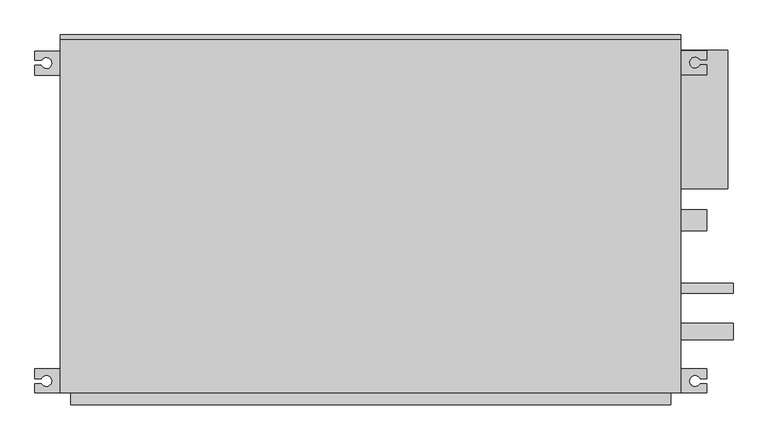
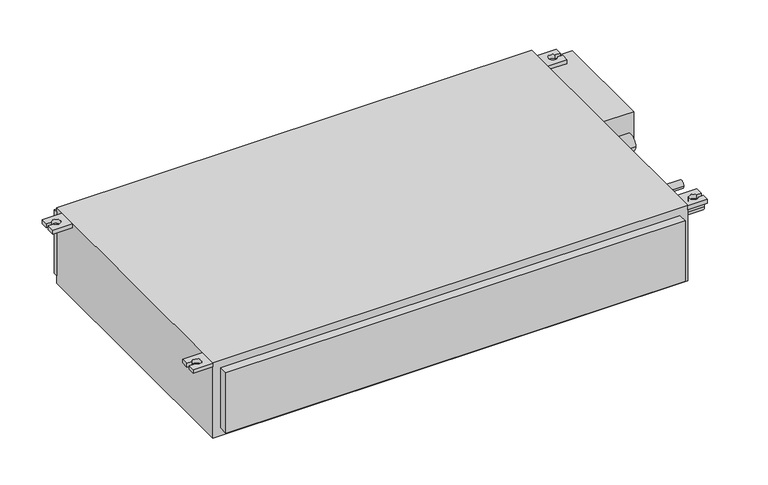
"""IFC4 building model written with IfcOpenShell, lengths in millimetres: proxy geometry, PEFY-P-NMSU-E_Low_Profile_Ducted : PEFY-P24NMSU-E."""

import ifcopenshell
import ifcopenshell.guid

model = None  # the IFC model being written
_history = None  # IfcOwnerHistory: only IFC2X3 demands one
_inside = {}  # id of a spatial element -> (the spatial element, [elements in it])
_under = {}  # id of a project, library or spatial element -> (it, [spatial elements below it])
_declared = {}  # id of a project -> (the project, [libraries it declares])
_typed = {}  # id of a type object -> (the type object, [elements of that type])
_made_of = {}  # id of a material, layer set ... -> (it, [elements and type objects made of it])


def new_model(schema):
    """Start an empty IFC model of exactly this schema.

    Asked for "IFC4X3", IfcOpenShell would pick the latest addendum, in which some entities
    have other attributes; the version numbers below select the first issue.
    IFC2X3 requires an IfcOwnerHistory on every rooted entity: one is made here for all.
    """
    global model, _history
    if schema == "IFC4X3":
        model = ifcopenshell.file(schema_version=(4, 3, 0, 0))
    else:
        model = ifcopenshell.file(schema=schema)
    _inside.clear()
    _under.clear()
    _declared.clear()
    _typed.clear()
    _made_of.clear()
    _history = None
    if model.schema == "IFC2X3":
        org = make("IfcOrganization", Name="unknown")
        user = make(
            "IfcPersonAndOrganization",
            ThePerson=make("IfcPerson", FamilyName="unknown"),
            TheOrganization=org,
        )
        app = make(
            "IfcApplication",
            ApplicationDeveloper=org,
            Version="unknown",
            ApplicationFullName="unknown",
            ApplicationIdentifier="unknown",
        )
        _history = make(
            "IfcOwnerHistory",
            OwningUser=user,
            OwningApplication=app,
            ChangeAction="ADDED",
            CreationDate=0,
        )
    return model


def make(cls, **values):
    """One entity of the class cls with the attributes given. An attribute that is None is left unset."""
    return model.create_entity(
        cls, **{name: value for name, value in values.items() if value is not None}
    )


def rooted(cls, **values):
    """An entity with a GlobalId (a new one), such as an element, a storey or a relation."""
    return make(cls, GlobalId=ifcopenshell.guid.new(), OwnerHistory=_history, **values)


def si_unit(unit_type, name, prefix=None):
    """IfcSIUnit, for example si_unit("LENGTHUNIT", "METRE", prefix="MILLI")."""
    return make("IfcSIUnit", UnitType=unit_type, Prefix=prefix, Name=name)


def assignment(units):
    """IfcUnitAssignment: the units of a project."""
    return None if units is None else make("IfcUnitAssignment", Units=units)


def point(xyz):
    """IfcCartesianPoint."""
    return None if xyz is None else make("IfcCartesianPoint", Coordinates=xyz)


def direction(xyz):
    """IfcDirection."""
    return None if xyz is None else make("IfcDirection", DirectionRatios=xyz)


def frame(location, z_axis=None, x_axis=None):
    """IfcAxis2Placement3D, a coordinate frame: its origin and axes. An axis left out is left unset."""
    return make(
        "IfcAxis2Placement3D",
        Location=point(location),
        Axis=direction(z_axis),
        RefDirection=direction(x_axis),
    )


def frame_2d(location, x_axis=None):
    """IfcAxis2Placement2D, a coordinate frame in the plane: its origin and x axis."""
    return make(
        "IfcAxis2Placement2D", Location=point(location), RefDirection=direction(x_axis)
    )


def origin():
    """The frame at (0, 0, 0) with its axes left unset."""
    return frame((0.0, 0.0, 0.0))


def origin_with_axes():
    """The frame at (0, 0, 0) with the z axis (0, 0, 1) and the x axis (1, 0, 0) written out."""
    return frame((0.0, 0.0, 0.0), z_axis=(0.0, 0.0, 1.0), x_axis=(1.0, 0.0, 0.0))


def place(relative_to, where):
    """IfcLocalPlacement: puts the frame where relative to a parent placement (None: the world)."""
    return make(
        "IfcLocalPlacement", PlacementRelTo=relative_to, RelativePlacement=where
    )


def context(
    kind, dimensions, precision=None, world=None, true_north=None, identifier=None
):
    """IfcGeometricRepresentationContext, for example the 3D "Model" context."""
    return make(
        "IfcGeometricRepresentationContext",
        ContextIdentifier=identifier,
        ContextType=kind,
        CoordinateSpaceDimension=dimensions,
        Precision=precision,
        WorldCoordinateSystem=world,
        TrueNorth=true_north,
    )


def project(units=None, contexts=None):
    """IfcProject with its units and contexts."""
    return rooted(
        "IfcProject",
        Name="project",
        RepresentationContexts=contexts,
        UnitsInContext=assignment(units),
    )


def spatial(cls, under=None, at=None, **own):
    """A site, building, storey or space (cls), placed at a placement, below another one or the project."""
    s = rooted(cls, ObjectPlacement=at, **own)
    if under is not None:
        _under.setdefault(under.id(), (under, []))[1].append(s)
    return s


def polyline(points):
    """IfcPolyline through the points."""
    return make("IfcPolyline", Points=[point(p) for p in points])


def circle_curve(where, radius):
    """IfcCircle in the frame where."""
    return make("IfcCircle", Position=where, Radius=radius)


def trimmed(basis, trim1, trim2, sense, master):
    """IfcTrimmedCurve: the piece of a basis curve between two trims."""
    return make(
        "IfcTrimmedCurve",
        BasisCurve=basis,
        Trim1=trim1,
        Trim2=trim2,
        SenseAgreement=sense,
        MasterRepresentation=master,
    )


def segment(curve, same_sense, transition):
    """IfcCompositeCurveSegment."""
    return make(
        "IfcCompositeCurveSegment",
        Transition=transition,
        SameSense=same_sense,
        ParentCurve=curve,
    )


def composite_curve(segments, self_intersect=None):
    """IfcCompositeCurve: segments joined end to end."""
    return make("IfcCompositeCurve", Segments=segments, SelfIntersect=self_intersect)


def outline(outer, holes=None, kind="AREA"):
    """IfcArbitraryClosedProfileDef: a profile drawn as a closed curve; with holes, ...WithVoids."""
    if holes is None:
        return make("IfcArbitraryClosedProfileDef", ProfileType=kind, OuterCurve=outer)
    return make(
        "IfcArbitraryProfileDefWithVoids",
        ProfileType=kind,
        OuterCurve=outer,
        InnerCurves=holes,
    )


def extrude(swept, where, along, depth):
    """IfcExtrudedAreaSolid: the profile swept, set in the frame where, extruded along a direction by depth."""
    return make(
        "IfcExtrudedAreaSolid",
        SweptArea=swept,
        Position=where,
        ExtrudedDirection=direction(along),
        Depth=depth,
    )


def shape(context_of_items, identifier, shape_type, items):
    """IfcShapeRepresentation: the items that make up one representation, for example the "Body"."""
    return make(
        "IfcShapeRepresentation",
        ContextOfItems=context_of_items,
        RepresentationIdentifier=identifier,
        RepresentationType=shape_type,
        Items=items,
    )


def source(mapping_origin, context_of_items, identifier, shape_type, items):
    """IfcRepresentationMap: a shape defined once, which mapped items show again and again."""
    return make(
        "IfcRepresentationMap",
        MappingOrigin=mapping_origin,
        MappedRepresentation=shape(context_of_items, identifier, shape_type, items),
    )


def transform(
    local_origin,
    x_axis=None,
    y_axis=None,
    z_axis=None,
    scale=None,
    scale2=None,
    scale3=None,
    uniform=True,
):
    """IfcCartesianTransformationOperator3D, or its non-uniform kind. x_axis, y_axis, z_axis: its Axis1, 2, 3."""
    if uniform:
        return make(
            "IfcCartesianTransformationOperator3D",
            Axis1=direction(x_axis),
            Axis2=direction(y_axis),
            LocalOrigin=point(local_origin),
            Scale=scale,
            Axis3=direction(z_axis),
        )
    return make(
        "IfcCartesianTransformationOperator3DnonUniform",
        Axis1=direction(x_axis),
        Axis2=direction(y_axis),
        LocalOrigin=point(local_origin),
        Scale=scale,
        Axis3=direction(z_axis),
        Scale2=scale2,
        Scale3=scale3,
    )


def mapped(mapping_source, mapping_target):
    """IfcMappedItem: shows the shape of a source again, moved by a transform."""
    return make(
        "IfcMappedItem", MappingSource=mapping_source, MappingTarget=mapping_target
    )


def made_of(thing, what):
    """Note that an element or type object is made of a material, layer set ...; save() writes the relation."""
    if what is not None:
        _made_of.setdefault(what.id(), (what, []))[1].append(thing)
    return thing


def element(
    cls,
    number,
    at=None,
    inside=None,
    cuts=None,
    type_object=None,
    material=None,
    context=None,
    identifier="Body",
    shape_type=None,
    held_by="IfcProductDefinitionShape",
    body=None,
    shapes=None,
    **own,
):
    """One element of the class cls, such as IfcWall. Its Tag is "e" and its number.

    at: its placement. inside: the storey or other place that contains it. cuts: it is an
    opening in that element (IfcRelVoidsElement). A single representation is given by context,
    identifier, shape_type and body (its items); several are given by shapes. held_by: the class
    of the entity that holds the representations. save() writes the other relations.
    """
    e = rooted(cls, Tag="e%d" % number, ObjectPlacement=at, **own)
    if body is not None:
        shapes = [shape(context, identifier, shape_type, body)]
    if shapes is not None:
        e.Representation = make(held_by, Representations=shapes)
    if inside is not None:
        _inside.setdefault(inside.id(), (inside, []))[1].append(e)
    if cuts is not None:
        rooted(
            "IfcRelVoidsElement", RelatingBuildingElement=cuts, RelatedOpeningElement=e
        )
    if type_object is not None:
        _typed.setdefault(type_object.id(), (type_object, []))[1].append(e)
    return made_of(e, material)


def aggregate(whole, parts):
    """IfcRelAggregates: a whole, such as a stair, and the parts it consists of."""
    return rooted("IfcRelAggregates", RelatingObject=whole, RelatedObjects=parts)


def save(model, path):
    """Write the relations noted so far, then the file.

    IfcRelAggregates (storeys below a building ...), IfcRelContainedInSpatialStructure (elements
    in a storey), IfcRelDefinesByType, IfcRelAssociatesMaterial and IfcRelDeclares: one each for
    every whole, place, type object, material and project.
    """
    for whole, parts in _under.values():
        aggregate(whole, parts)
    for where, things in _inside.values():
        rooted(
            "IfcRelContainedInSpatialStructure",
            RelatedElements=things,
            RelatingStructure=where,
        )
    for kind, things in _typed.values():
        rooted("IfcRelDefinesByType", RelatedObjects=things, RelatingType=kind)
    for what, things in _made_of.values():
        rooted("IfcRelAssociatesMaterial", RelatedObjects=things, RelatingMaterial=what)
    for by, libraries in _declared.values():
        rooted("IfcRelDeclares", RelatingContext=by, RelatedDefinitions=libraries)
    model.write(path)


def mechanical_equipment_2ac3c092(model_context):
    return source(origin(), model_context, "Body", "SweptSolid", [
        extrude(outline(composite_curve([segment(polyline([(-644.3, 282.0), (-644.3, 300.9759165), (-632.1454311, 300.9759165)]), True, "CONTINUOUS"), segment(trimmed(circle_curve(frame_2d((-622.2863556, 305.4254582)), 10.8166442), [point((-632.1454311, 300.9759165))], [point((-631.8387803, 310.5))], True, "CARTESIAN"), True, "CONTINUOUS"), segment(polyline([(-631.8387803, 310.5), (-644.3, 310.5), (-644.3, 328.0), (-595.3, 328.0), (-595.3, 282.0), (-644.3, 282.0)]), True, "CONTINUOUS")], self_intersect=False)), frame((0.0, 0.0, 188.55), z_axis=(0.0, 0.0, 1.0), x_axis=(1.0, 0.0, 0.0)), (0.0, 0.0, 1.0), 10.0),
        extrude(outline(composite_curve([segment(polyline([(-644.3, -281.0), (-595.3, -281.0), (-595.3, -327.0), (-644.3, -327.0), (-644.3, -309.5), (-631.8387803, -309.5)]), True, "CONTINUOUS"), segment(trimmed(circle_curve(frame_2d((-622.2863556, -304.4254582)), 10.8166442), [point((-631.8387803, -309.5))], [point((-632.1454311, -299.9759165))], True, "CARTESIAN"), True, "CONTINUOUS"), segment(polyline([(-632.1454311, -299.9759165), (-644.3, -299.9759165), (-644.3, -281.0)]), True, "CONTINUOUS")], self_intersect=False)), frame((0.0, 0.0, 188.55), z_axis=(0.0, 0.0, 1.0), x_axis=(1.0, 0.0, 0.0)), (0.0, 0.0, 1.0), 10.0),
        extrude(outline(composite_curve([segment(polyline([(644.3, 282.9429009), (595.3, 282.9429009), (595.3, 328.9429009), (644.3, 328.9429009), (644.3, 311.4429009), (631.8387803, 311.4429009)]), True, "CONTINUOUS"), segment(trimmed(circle_curve(frame_2d((622.2863556, 306.3683591)), 10.8166442), [point((631.8387803, 311.4429009))], [point((632.1454311, 301.9188174))], True, "CARTESIAN"), True, "CONTINUOUS"), segment(polyline([(632.1454311, 301.9188174), (644.3, 301.9188174), (644.3, 282.9429009)]), True, "CONTINUOUS")], self_intersect=False)), frame((0.0, 0.0, 188.55), z_axis=(0.0, 0.0, 1.0), x_axis=(1.0, 0.0, 0.0)), (0.0, 0.0, 1.0), 10.0),
        extrude(outline(composite_curve([segment(polyline([(644.3, -281.0), (644.3, -299.9759165), (632.1454311, -299.9759165)]), True, "CONTINUOUS"), segment(trimmed(circle_curve(frame_2d((622.2863556, -304.4254582)), 10.8166442), [point((632.1454311, -299.9759165))], [point((631.8387803, -309.5))], True, "CARTESIAN"), True, "CONTINUOUS"), segment(polyline([(631.8387803, -309.5), (644.3, -309.5), (644.3, -327.0), (595.3, -327.0), (595.3, -281.0), (644.3, -281.0)]), True, "CONTINUOUS")], self_intersect=False)), frame((0.0, 0.0, 188.55), z_axis=(0.0, 0.0, 1.0), x_axis=(1.0, 0.0, 0.0)), (0.0, 0.0, 1.0), 10.0),
        extrude(outline(polyline([(595.3, 350.04375), (-595.3, 350.04375), (-595.3, 359.5477547), (595.3, 359.5477547), (595.3, 350.04375)])), frame((0.0, 0.0, 20.0), z_axis=(0.0, 0.0, 1.0), x_axis=(1.0, 0.0, 0.0)), (0.0, 0.0, 1.0), 168.55),
        extrude(outline(composite_curve([segment(trimmed(circle_curve(frame_2d((4.0570991, 59.8)), 20.0), [point((-15.9429009, 59.8))], [point((24.0570991, 59.8))], False, "CARTESIAN"), True, "CONTINUOUS"), segment(trimmed(circle_curve(frame_2d((4.0570991, 59.8)), 20.0), [point((24.0570991, 59.8))], [point((-15.9429009, 59.8))], False, "CARTESIAN"), True, "CONTINUOUS")], self_intersect=False)), frame((595.3, 0.0, 0.0), z_axis=(1.0, 0.0, 0.0), x_axis=(0.0, 1.0, 0.0)), (0.0, 0.0, 1.0), 26.9863556),
        extrude(outline(composite_curve([segment(trimmed(circle_curve(frame_2d((4.0570991, 149.6)), 20.0), [point((-15.9429009, 149.6))], [point((24.0570991, 149.6))], False, "CARTESIAN"), True, "CONTINUOUS"), segment(trimmed(circle_curve(frame_2d((4.0570991, 149.6)), 20.0), [point((24.0570991, 149.6))], [point((-15.9429009, 149.6))], False, "CARTESIAN"), True, "CONTINUOUS")], self_intersect=False)), frame((595.3, 0.0, 0.0), z_axis=(1.0, 0.0, 0.0), x_axis=(0.0, 1.0, 0.0)), (0.0, 0.0, 1.0), 49.0),
        extrude(outline(composite_curve([segment(trimmed(circle_curve(frame_2d((-126.5596979, 100.0)), 9.5), [point((-136.0596979, 100.0))], [point((-117.0596979, 100.0))], False, "CARTESIAN"), True, "CONTINUOUS"), segment(trimmed(circle_curve(frame_2d((-126.5596979, 100.0)), 9.5), [point((-117.0596979, 100.0))], [point((-136.0596979, 100.0))], False, "CARTESIAN"), True, "CONTINUOUS")], self_intersect=False)), frame((595.3, 0.0, 0.0), z_axis=(1.0, 0.0, 0.0), x_axis=(0.0, 1.0, 0.0)), (0.0, 0.0, 1.0), 100.0),
        extrude(outline(composite_curve([segment(trimmed(circle_curve(frame_2d((-209.7540575, 100.0)), 15.9), [point((-225.6540575, 100.0))], [point((-193.8540575, 100.0))], False, "CARTESIAN"), True, "CONTINUOUS"), segment(trimmed(circle_curve(frame_2d((-209.7540575, 100.0)), 15.9), [point((-193.8540575, 100.0))], [point((-225.6540575, 100.0))], False, "CARTESIAN"), True, "CONTINUOUS")], self_intersect=False)), frame((595.3, 0.0, 0.0), z_axis=(1.0, 0.0, 0.0), x_axis=(0.0, 1.0, 0.0)), (0.0, 0.0, 1.0), 100.0),
        extrude(outline(polyline([(685.3, 330.0), (685.3, 64.0570991), (595.3, 64.0570991), (595.3, 330.0), (685.3, 330.0)])), frame((0.0, 0.0, 20.0), z_axis=(0.0, 0.0, 1.0), x_axis=(1.0, 0.0, 0.0)), (0.0, 0.0, 1.0), 159.8),
        extrude(outline(polyline([(575.3, -350.04375), (-575.3, -350.04375), (-575.3, -327.0), (575.3, -327.0), (575.3, -350.04375)])), frame((0.0, 0.0, 20.0), z_axis=(0.0, 0.0, 1.0), x_axis=(1.0, 0.0, 0.0)), (0.0, 0.0, 1.0), 159.8),
        extrude(outline(polyline([(-595.3, -327.0), (-595.3, 350.04375), (595.3, 350.04375), (595.3, -327.0), (-595.3, -327.0)])), origin_with_axes(), (0.0, 0.0, 1.0), 200.0),
    ])


if __name__ == "__main__":
    model = new_model("IFC4")
    model_context = context("Model", 3, world=origin())
    ifc_project = project(units=[si_unit("LENGTHUNIT", "METRE", prefix="MILLI")], contexts=[model_context])
    site = spatial("IfcSite", under=ifc_project)
    building = spatial("IfcBuilding", under=site)
    placement = place(None, origin())
    mechanical_equipment_shape = mechanical_equipment_2ac3c092(model_context)
    element("IfcBuildingElementProxy", 1, Name="PEFY-P-NMSU-E_Low_Profile_Ducted : PEFY-P24NMSU-E", ObjectType="PEFY-P-NMSU-E_Low_Profile_Ducted : PEFY-P24NMSU-E", at=placement, inside=building, context=model_context, shape_type="MappedRepresentation", body=[
        mapped(mechanical_equipment_shape, transform((0.0, 0.0, 0.0), x_axis=(1.0, 0.0, 0.0), y_axis=(0.0, 1.0, 0.0), z_axis=(0.0, 0.0, 1.0))),
    ])
    save(model, "model.ifc")

# Revit data of these elements
# Project information
#   Project Issue Date = "Issue Date"
#   Project Status = "Project Status"
#   Client Name = "Owner"
#   Project Address = "Enter address here"
#   Project Name = "Project Name"
#   Project Number = "Project Number"
# Type "PEFY-P-NMSU-E_Low_Profile_Ducted : PEFY-P24NMSU-E"
#   Subcategory = "HVAC"
#   Standard Air Filter = "Polypropylene Honeycomb"
#   Specification URL = "http://www.mrslim.com/customerCare/resources.asp"
#   Sound Pressure Levels (dB(A)) = "30-35-40"
#   SmartBIM Object Created By = "Reed Construction Data"
#   Refirigerant Pipe diameter (Liquid) = "3/8\""
#   Refirigerant Pipe diameter (Gas) = "5/8\""
#   Power Source = "208/230, 1, 60"
#   Power Consumption Heating = "0.10 kW"
#   Power Consumption Cooling = "0.12 kW"
#   Unit Weight (LBS) = "62"
#   Model = "PEFY-P24NMSU-E"
#   Manufacturer URL = "http://www.mrslim.com/customerCare/resources.asp"
#   Manufacturer = "Mitsubishi Electric"
#   Installation URL = "http://www.mrslim.com/customerCare/resources.asp"
#   Fan Motor Type = "DC Motor"
#   Fan Motor Output = "0.096 kW"
#   MCA = "1.57/1.73"
#   MOCP = "15 A"
#   E.S.P (In. W.G.) = ".02-.20"
#   Drainpipe Dimension = "1-1/4"
#   Description = "Ceiling Concealed Ducted Low Profile"
#   Condensate Lift Mechanism = "21-11/16\""
#   Coil Type = "Cross Fin"
#   Heating Capacity (BTU) = "27000"
#   Fan Type x Quantity = "Sirocco Fan x 2"
#   Current Heating = "0.83 A"
#   Current Cooling = "0.93 A"
#   Cooling Capacity (BTU) = "24000"
#   Fan capacity (CFM) = "423-565-706"
#   Assembly Code = "D3050200"
#   95 CSI = "15760"
#   04 CSI = "23 82 19 "
#   Width = 3' - 10.87402"
#   Voltage = 208 V
#   Unit Supply Airflow [instance default] = 390 CFM
#   Unit Return Airflow [instance default] = 390 CFM
#   SmartBIM Object Version = 3
#   Height = 0' - 7.87402"
#   Drain Pipe Radius = 0' - 0.7874"
#   Depth = 2' - 3 9/16"
#   Default Elevation = 4' - 0"
#   C = 4' - 2.73228"
#   Brazing Connection Radius (Liquid) = 0' - 0.37402"
#   Brazing Connection Radius (Gas) = 0' - 0.62598"
#   Suspension Bolt Pitch = 4' - 0.92126"
#   Apparent Load = 0 VA
#   Air Outlet Width = 3' - 9.29921"
#   Air Inlet Width = 3' - 10.87402"
#   Air Outlet Height = 0' - 6.29134"
#   Air Inlet Height = 0' - 6.65354"
#   Number of Poles = 1
#   Load Classification = Other
#   External Finish = Galvanized Steel Sheet
#   Air Outlet Unit Material = Metal Grill
#   Air Inlet Unit Material = Grill
#   URL = ""
# Element 1 (IfcBuildingElementProxy, "PEFY-P-NMSU-E_Low_Profile_Ducted : PEFY-P24NMSU-E")
#   Unit Supply Airflow = 300 CFM
#   Unit Return Airflow = 0 CFM
#   Materials on its faces: "Galvanized Steel Sheet", "Grill", "Metal Grill"
# Materials
#   "Galvanized Steel Sheet": class "Metal", colour RGB 189 187 185, transparency 0
#   "Metal Grill": class "Metal", colour RGB 10 10 10, transparency 0
#   "Grill": class "Plastic", colour RGB 5 5 5, transparency 0
